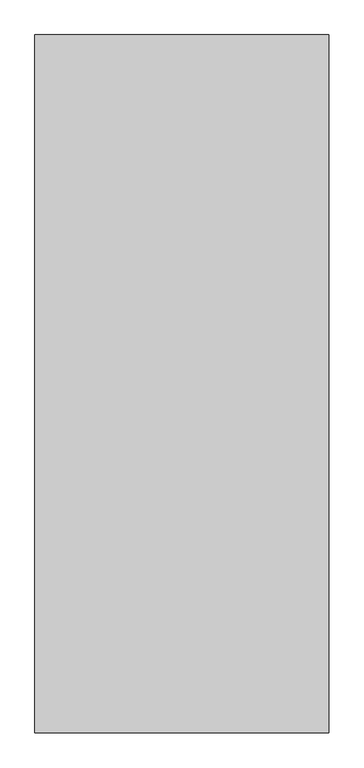
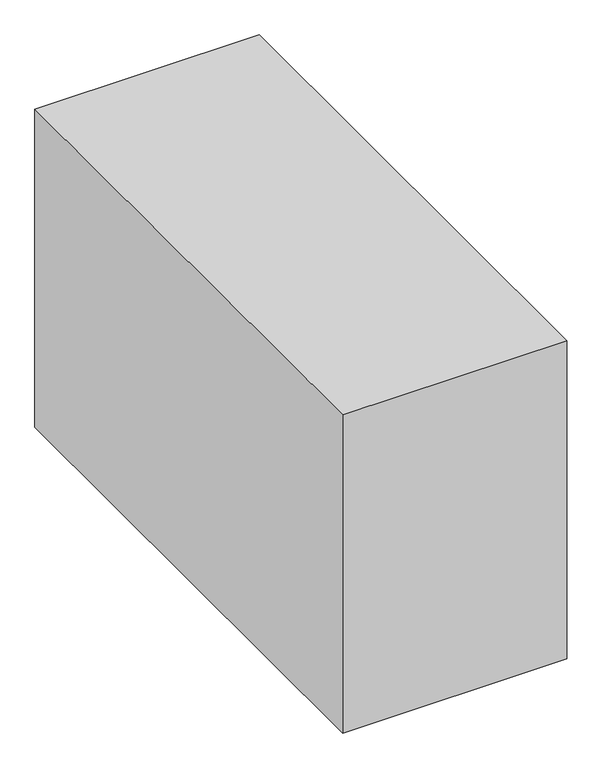
"""IFC4 building model written with IfcOpenShell, lengths in millimetres: proxy geometry, Space Planning Box_hec : Space Planning Box_hec."""

from ifc_helpers import new_model, si_unit, origin, origin_with_axes, place, context, project, spatial, polyline, outline, extrude, source, transform, mapped, element, save


def generic_models_3a820573(model_context):
    return source(origin(), model_context, "Body", "SweptSolid", [
        extrude(outline(polyline([(2000.0, 4750.0), (2000.0, -4750.0), (-2000.0, -4750.0), (-2000.0, 4750.0), (2000.0, 4750.0)])), origin_with_axes(), (0.0, 0.0, 1.0), 6000.0),
    ])


if __name__ == "__main__":
    model = new_model("IFC4")
    model_context = context("Model", 3, world=origin())
    ifc_project = project(units=[si_unit("LENGTHUNIT", "METRE", prefix="MILLI")], contexts=[model_context])
    site = spatial("IfcSite", under=ifc_project)
    building = spatial("IfcBuilding", under=site)
    placement = place(None, origin())
    generic_models_shape = generic_models_3a820573(model_context)
    element("IfcBuildingElementProxy", 1, Name="Space Planning Box_hec : Space Planning Box_hec", ObjectType="Space Planning Box_hec : Space Planning Box_hec", at=placement, inside=building, context=model_context, shape_type="MappedRepresentation", body=[
        mapped(generic_models_shape, transform((0.0, 0.0, 0.0), x_axis=(1.0, 0.0, 0.0), y_axis=(0.0, 1.0, 0.0), z_axis=(0.0, 0.0, 1.0))),
    ])
    save(model, "model.ifc")

# Revit data of these elements
# Type "Space Planning Box_hec : Space Planning Box_hec"
#   Type Comments = "..."
#   Room Name [instance default] = "?"
#   Interior Finish [instance default] = ""
#   Exterior Finish [instance default] = ""
#   Department [instance default] = ""
#   Assembly Code = "..."
#   Width [instance default] = 1524 mm
#   Program Area [instance default] = 0.00 m²
#   Length [instance default] = 1524 mm
#   Height [instance default] = 1524 mm
#   Area [instance default] = 2.32258 m²
#   Fill Color [instance default] = Cyan
#   Default Elevation = 0
# Element 1 (IfcBuildingElementProxy, "Space Planning Box_hec : Space Planning Box_hec")
#   Room Name = "Stairway"
#   Interior Finish = "IF2"
#   Exterior Finish = "EF1"
#   Department = "AR"
#   Width = 4000 mm
#   Program Area = 38.00 m²
#   Length = 9500 mm
#   Height = 6000 mm
#   Area = 38.00 m²
#   Materials on its faces: "Cyan"
# Materials
#   "Cyan": class "Generic", colour RGB 0 255 255, transparency 0.2, Cost = 0
